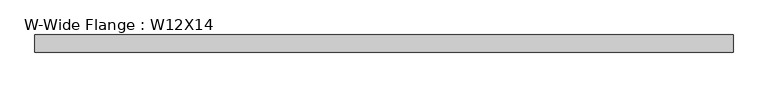
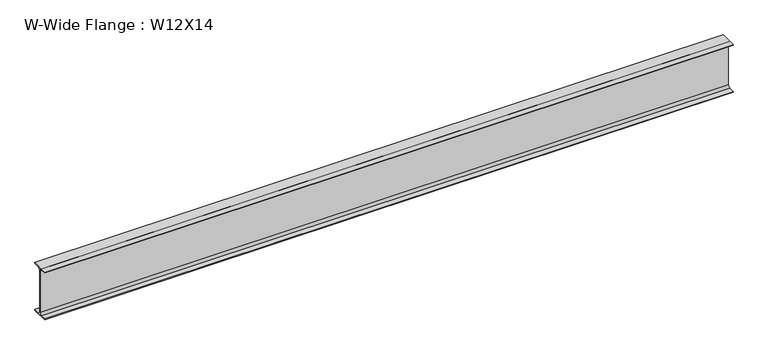
"""IFC4 building model written with IfcOpenShell, lengths in millimetres: beam geometry, W-Wide Flange : W12X14."""

from ifc_helpers import new_model, si_unit, point, frame, frame_2d, origin, place, context, project, spatial, polyline, circle_curve, trimmed, segment, composite_curve, outline, extrude, source, transform, mapped, element, save


def w_wide_flange_w12x14_025fe0ad(model_context):
    return source(origin(), model_context, "Body", "SweptSolid", [
        extrude(outline(composite_curve([segment(polyline([(50.419, -145.415), (50.419, -151.13), (-50.419, -151.13), (-50.419, -145.415), (-15.875, -145.415)]), True, "CONTINUOUS"), segment(trimmed(circle_curve(frame_2d((-15.875, -132.08)), 13.335), [point((-15.875, -145.415))], [point((-2.54, -132.08))], True, "CARTESIAN"), True, "CONTINUOUS"), segment(polyline([(-2.54, -132.08), (-2.54, 132.08)]), True, "CONTINUOUS"), segment(trimmed(circle_curve(frame_2d((-15.875, 132.08)), 13.335), [point((-2.54, 132.08))], [point((-15.875, 145.415))], True, "CARTESIAN"), True, "CONTINUOUS"), segment(polyline([(-15.875, 145.415), (-50.419, 145.415), (-50.419, 151.13), (50.419, 151.13), (50.419, 145.415), (15.875, 145.415)]), True, "CONTINUOUS"), segment(trimmed(circle_curve(frame_2d((15.875, 132.08)), 13.335), [point((15.875, 145.415))], [point((2.54, 132.08))], True, "CARTESIAN"), True, "CONTINUOUS"), segment(polyline([(2.54, 132.08), (2.54, -132.08)]), True, "CONTINUOUS"), segment(trimmed(circle_curve(frame_2d((15.875, -132.08)), 13.335), [point((2.54, -132.08))], [point((15.875, -145.415))], True, "CARTESIAN"), True, "CONTINUOUS"), segment(polyline([(15.875, -145.415), (50.419, -145.415)]), True, "CONTINUOUS")], self_intersect=False)), frame((-2032.0, 0.0, 0.0), z_axis=(1.0, 0.0, 0.0), x_axis=(0.0, 1.0, 0.0)), (0.0, 0.0, 1.0), 4114.8),
    ])


if __name__ == "__main__":
    model = new_model("IFC4")
    model_context = context("Model", 3, world=origin())
    ifc_project = project(units=[si_unit("LENGTHUNIT", "METRE", prefix="MILLI")], contexts=[model_context])
    site = spatial("IfcSite", under=ifc_project)
    building = spatial("IfcBuilding", under=site)
    placement = place(None, origin())
    w_wide_flange_w12x14_shape = w_wide_flange_w12x14_025fe0ad(model_context)
    element("IfcBeam", 1, ObjectType="W-Wide Flange : W12X14", at=placement, inside=building, context=model_context, shape_type="MappedRepresentation", body=[
        mapped(w_wide_flange_w12x14_shape, transform((0.0, 0.0, 0.0), x_axis=(1.0, 0.0, 0.0), y_axis=(0.0, 1.0, 0.0), z_axis=(0.0, 0.0, 1.0))),
    ])
    save(model, "model.ifc")

# Revit data of these elements
# Type "W-Wide Flange : W12X14"
#   Assembly Code = "B10"
#   W = 14
#   Length [instance default] = 5' - 0"
#   bf = 0' - 3.97"
#   d = 0' - 11.9"
#   k = 0' - 0 3/4"
#   k2 = 0' - 0.525"
#   tf = 0' - 0.225"
#   tw = 0' - 0.2"
#   A = 0.0288889 SF
#   Structural Material [instance default] = Steel ASTM A992
# Element 1 (IfcBeam, "W-Wide Flange : W12X14")
#   Materials on its faces: "Steel ASTM A992"
# Materials
#   "Steel ASTM A992": class "Metal", colour RGB 199 199 199, transparency 0, Description = "Structural steel 50ksi", Cost = 0
